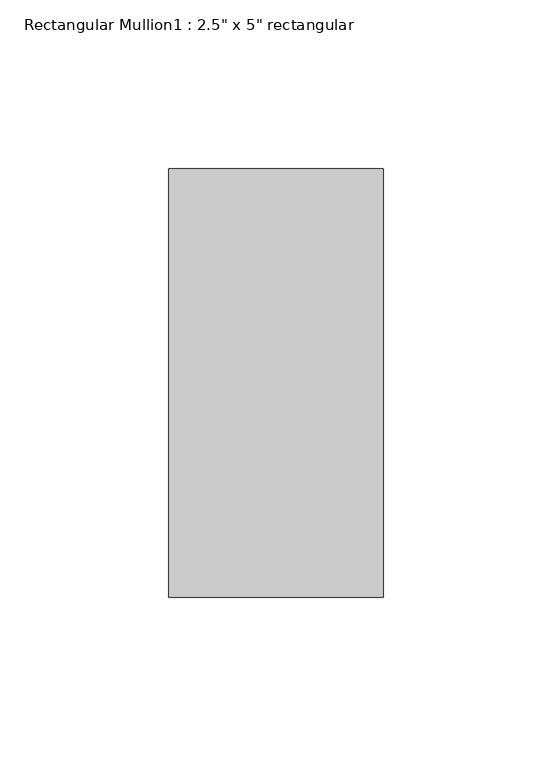
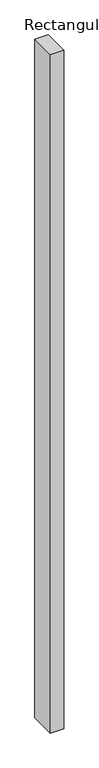
"""IFC4 building model written with IfcOpenShell, lengths in millimetres: member geometry."""

from ifc_helpers import new_model, si_unit, frame, origin, place, context, project, spatial, polyline, outline, extrude, source, transform, mapped, element, save


def member_9434a11c(model_context):
    return source(origin(), model_context, "Body", "SweptSolid", [
        extrude(outline(polyline([(0.0, 63.5), (0.0, -63.5), (-63.5, -63.5), (-63.5, 63.5), (0.0, 63.5)])), frame((0.0, 0.0, -3382.4333333), z_axis=(0.0, 0.0, 1.0), x_axis=(1.0, 0.0, 0.0)), (0.0, 0.0, 1.0), 3382.4333333),
    ])


if __name__ == "__main__":
    model = new_model("IFC4")
    model_context = context("Model", 3, world=origin())
    ifc_project = project(units=[si_unit("LENGTHUNIT", "METRE", prefix="MILLI")], contexts=[model_context])
    site = spatial("IfcSite", under=ifc_project)
    building = spatial("IfcBuilding", under=site)
    placement = place(None, origin())
    member_shape = member_9434a11c(model_context)
    element("IfcMember", 1, ObjectType="Rectangular Mullion1 : 2.5\" x 5\" rectangular", at=placement, inside=building, context=model_context, shape_type="MappedRepresentation", body=[
        mapped(member_shape, transform((0.0, 0.0, 0.0), x_axis=(1.0, 0.0, 0.0), y_axis=(0.0, 1.0, 0.0), z_axis=(0.0, 0.0, 1.0))),
    ])
    save(model, "model.ifc")

# Revit data of these elements
# Type "Rectangular Mullion1 : 2.5\" x 5\" rectangular"
#   built-in parameter 1007304 = 0.416667 (stored number, unit not read)
#   built-in parameter 1007301 = 0.104167 (stored number, unit not read)
#   built-in parameter 1007300 = 0.104167 (stored number, unit not read)
# Element 1 (IfcMember, "Rectangular Mullion1 : 2.5\" x 5\" rectangular")
#   Materials on its faces: "support-frame"
# Materials
#   "support-frame": class "Unassigned", colour RGB 233 233 233, transparency 0, Cost = 0
